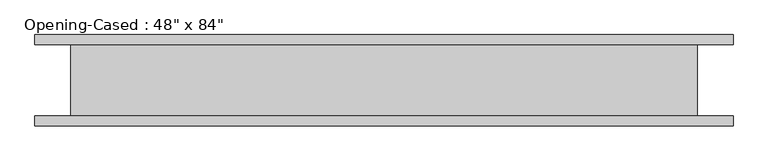
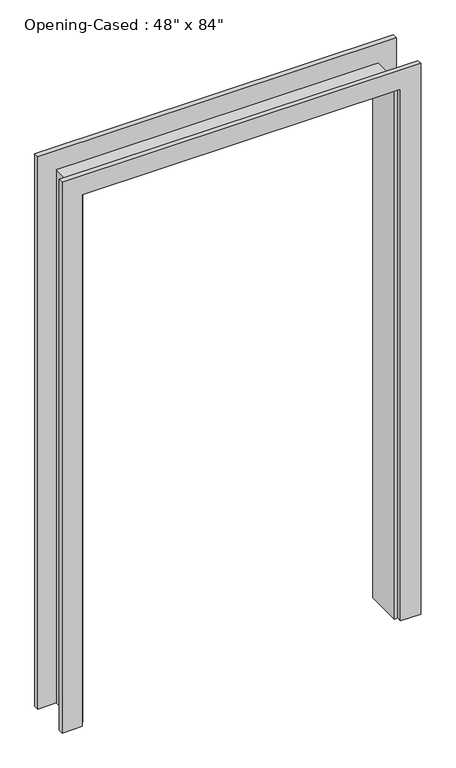
"""IFC4 building model written with IfcOpenShell, lengths in millimetres: proxy geometry."""

from ifc_helpers import new_model, si_unit, frame, origin, place, context, project, spatial, polyline, outline, extrude, faceted_brep, source, transform, mapped, element, save


def proxy_50e7bca7(model_context):
    return source(origin(), model_context, "Body", "SolidModel", [
        extrude(outline(polyline([(0.0, -611.4386567), (2127.25, -611.4386567), (2127.25, 595.0613433), (0.0, 595.0613433), (0.0, 671.2613433), (2203.45, 671.2613433), (2203.45, -687.6386567), (0.0, -687.6386567), (0.0, -611.4386567)])), frame((0.0, -88.9, 0.0), z_axis=(0.0, 1.0, 0.0), x_axis=(0.0, 0.0, 1.0)), (0.0, 0.0, 1.0), 19.05),
        extrude(outline(polyline([(0.0, 671.2613433), (2209.8, 671.2613433), (2209.8, -687.6386567), (0.0, -687.6386567), (0.0, -611.4386567), (2127.25, -611.4386567), (2127.25, 595.0613433), (0.0, 595.0613433), (0.0, 671.2613433)])), frame((0.0, 69.85, 0.0), z_axis=(0.0, 1.0, 0.0), x_axis=(0.0, 0.0, 1.0)), (0.0, 0.0, 1.0), 19.05),
        faceted_brep([(582.3613433, 69.85, 0.0), (601.4113433, 69.85, 0.0), (601.4113433, -69.85, 0.0), (582.3613433, -69.85, 0.0), (582.3613433, 69.85, 2114.55), (601.4113433, 69.85, 2133.6), (601.4113433, -69.85, 2133.6), (582.3613433, -69.85, 2114.55), (-598.7386567, 69.85, 2114.55), (-617.7886567, 69.85, 2133.6), (-617.7886567, -69.85, 2133.6), (-598.7386567, -69.85, 2114.55), (-598.7386567, 69.85, 0.0), (-598.7386567, -69.85, 0.0), (-617.7886567, -69.85, 0.0), (-617.7886567, 69.85, 0.0)], [[[0, 1, 2, 3]], [[1, 0, 4, 5]], [[2, 1, 5, 6]], [[3, 2, 6, 7]], [[0, 3, 7, 4]], [[5, 4, 8, 9]], [[6, 5, 9, 10]], [[7, 6, 10, 11]], [[4, 7, 11, 8]], [[12, 13, 14, 15]], [[9, 8, 12, 15]], [[10, 9, 15, 14]], [[11, 10, 14, 13]], [[8, 11, 13, 12]]]),
    ])


if __name__ == "__main__":
    model = new_model("IFC4")
    model_context = context("Model", 3, world=origin())
    ifc_project = project(units=[si_unit("LENGTHUNIT", "METRE", prefix="MILLI")], contexts=[model_context])
    site = spatial("IfcSite", under=ifc_project)
    building = spatial("IfcBuilding", under=site)
    placement = place(None, origin())
    proxy_shape = proxy_50e7bca7(model_context)
    element("IfcBuildingElementProxy", 1, Name="Opening-Cased : 48\" x 84\"", ObjectType="Opening-Cased : 48\" x 84\"", at=placement, inside=building, context=model_context, shape_type="MappedRepresentation", body=[
        mapped(proxy_shape, transform((0.0, 0.0, 0.0), x_axis=(1.0, 0.0, 0.0), y_axis=(0.0, 1.0, 0.0), z_axis=(0.0, 0.0, 1.0))),
    ])
    save(model, "model.ifc")

# Revit data of these elements
# Type "Opening-Cased : 48\" x 84\""
#   Height = 7' - 0"
#   Trim Thickness = 0' - 0 3/4"
#   Trim Width = 0' - 3"
#   Width = 4' - 0"
#   Frame Material = Door - Frame
#   Assembly Code = ""
# Element 1 (IfcBuildingElementProxy, "Opening-Cased : 48\" x 84\"")
#   Materials on its faces: "Door - Frame"
# Materials
#   "Door - Frame": class "Unassigned", colour RGB 118 70 51, transparency 0, Comments = "Rendering appearance not upgraded Rendering appearance not upgraded "
